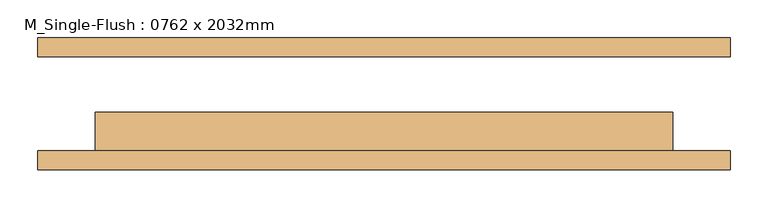
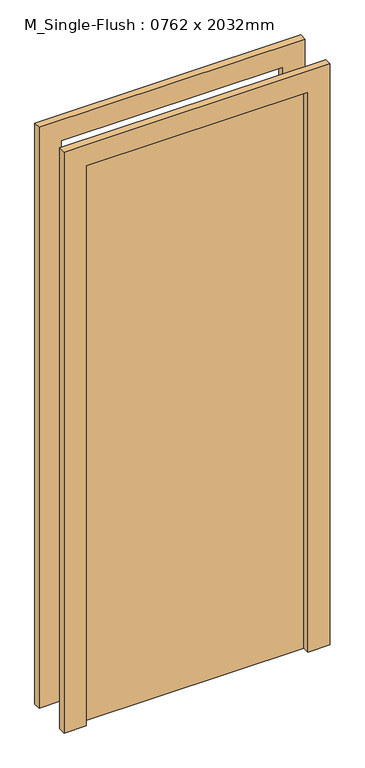
"""IFC4 building model written with IfcOpenShell, lengths in millimetres: door geometry, M_Single-Flush : 0762 x 2032mm."""

from ifc_helpers import new_model, si_unit, frame, origin, origin_with_axes, place, context, project, spatial, polyline, outline, extrude, source, transform, mapped, element, save


def m_single_flush_0762_x_2032mm_1c354163(model_context):
    return source(origin(), model_context, "Body", "SweptSolid", [
        extrude(outline(polyline([(2108.0, -457.0), (0.0, -457.0), (0.0, -381.0), (2032.0, -381.0), (2032.0, 381.0), (0.0, 381.0), (0.0, 457.0), (2108.0, 457.0), (2108.0, -457.0)])), frame((0.0, -87.0, 0.0), z_axis=(0.0, 1.0, 0.0), x_axis=(0.0, 0.0, 1.0)), (0.0, 0.0, 1.0), 25.0),
        extrude(outline(polyline([(2108.0, 457.0), (2108.0, -457.0), (0.0, -457.0), (0.0, -381.0), (2032.0, -381.0), (2032.0, 381.0), (0.0, 381.0), (0.0, 457.0), (2108.0, 457.0)])), frame((0.0, 62.0, 0.0), z_axis=(0.0, 1.0, 0.0), x_axis=(0.0, 0.0, 1.0)), (0.0, 0.0, 1.0), 25.0),
        extrude(outline(polyline([(381.0, -11.0), (381.0, -62.0), (-381.0, -62.0), (-381.0, -11.0), (381.0, -11.0)])), origin_with_axes(), (0.0, 0.0, 1.0), 2032.0),
    ])


if __name__ == "__main__":
    model = new_model("IFC4")
    model_context = context("Model", 3, world=origin())
    ifc_project = project(units=[si_unit("LENGTHUNIT", "METRE", prefix="MILLI")], contexts=[model_context])
    site = spatial("IfcSite", under=ifc_project)
    building = spatial("IfcBuilding", under=site)
    placement = place(None, origin())
    m_single_flush_0762_x_2032mm_shape = m_single_flush_0762_x_2032mm_1c354163(model_context)
    element("IfcDoor", 1, ObjectType="M_Single-Flush : 0762 x 2032mm", at=placement, inside=building, context=model_context, shape_type="MappedRepresentation", body=[
        mapped(m_single_flush_0762_x_2032mm_shape, transform((0.0, 0.0, 0.0), x_axis=(1.0, 0.0, 0.0), y_axis=(0.0, 1.0, 0.0), z_axis=(0.0, 0.0, 1.0))),
    ])
    save(model, "model.ifc")

# Revit data of these elements
# Type "M_Single-Flush : 0762 x 2032mm"
#   Manufacturer = "Manufacturer"
#   Type Mark = "28"
#   Construction Type = "Construction Type"
#   Fire Rating = "Fire Rating"
#   AccessibilityPerformance = "AccessibilityPerformance"
#   CodePerformance = "CodePerformance"
#   IsFireExit = "IsFireExit"
#   ConstructionType = "ConstructionType"
#   GlazingAreaFraction = "GlazingAreaFraction"
#   OperationType = "OperationType"
#   Area = "Area"
#   Color = "Color"
#   Constituents = "Constituents"
#   Features = "Features"
#   Finish = "Finish"
#   Grade = "Grade"
#   Material = "Material"
#   ModelReference = "ModelReference"
#   NominalHeight = "NominalHeight"
#   NominalLength = "NominalLength"
#   NominalWidth = "NominalWidth"
#   ProductionYear = "ProductionYear"
#   Reference = "Reference"
#   Shape = "Shape"
#   Size = "Size"
#   SustainabilityPerformance = "SustainabilityPerformance"
#   WarrantyDescription = "WarrantyDescription"
#   WarrantyDurationLabor = "WarrantyDurationLabor"
#   WarrantyDurationParts = "WarrantyDurationParts"
#   WarrantyGuarantorLabor = "WarrantyGuarantorLabor"
#   WarrantyGuarantorParts = "WarrantyGuarantorParts"
#   ExpectedLife = "ExpectedLife"
#   ReplacementCost = "ReplacementCost"
#   AssetAccountingType = "FIXED"
#   ModelLabel = "ModelLabel"
#   Thickness = 0.051 m
#   Height = 2.032 m
#   Trim Projection Ext = 0.025 m
#   Trim Projection Int = 0.025 m
#   Trim Width = 0.076 m
#   Width = 0.762 m
#   Door Material = Door - Panel
#   Frame Material = Door - Frame
#   Function = (empty or 0)
#   Wall Closure = (empty or 0)
# Element 1 (IfcDoor, "M_Single-Flush : 0762 x 2032mm")
#   Materials on its faces: "Door - Frame", "Door - Panel"
# Materials
#   "Door - Panel": class "Wood", colour RGB 210 159 95, transparency 0
#   "Door - Frame": class "Miscellaneous", colour RGB 118 70 51, transparency 0
